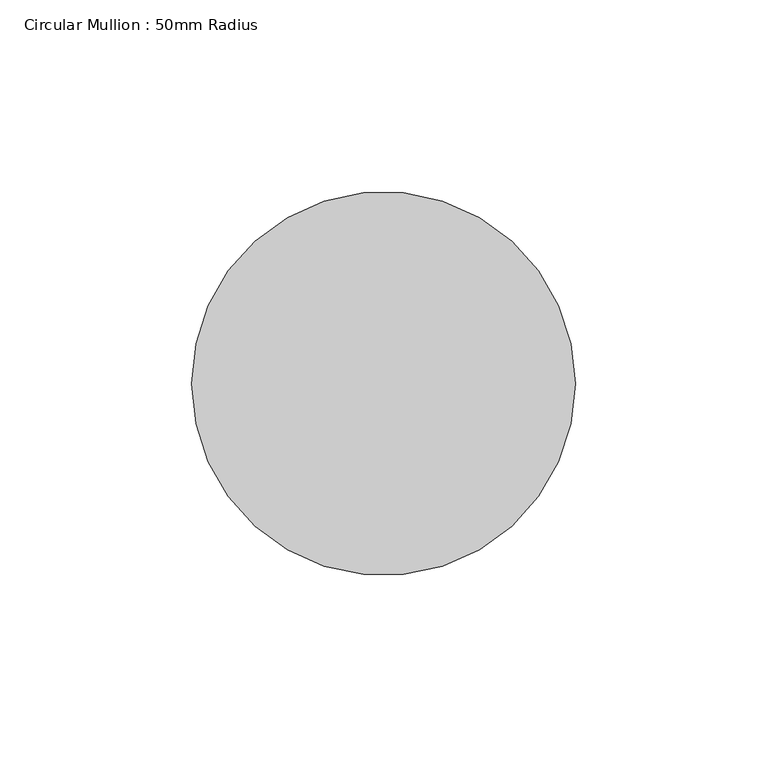
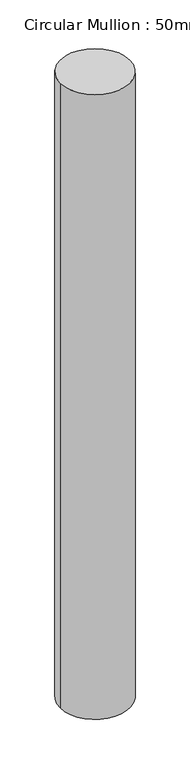
"""IFC4 building model written with IfcOpenShell, lengths in millimetres: member geometry, Circular Mullion : 50mm Radius."""

from ifc_helpers import new_model, si_unit, point, frame, origin, origin_2d, place, context, project, spatial, circle_curve, trimmed, segment, composite_curve, outline, extrude, source, transform, mapped, element, save


def circular_mullion_50mm_radius_479e7c5f(model_context):
    return source(origin(), model_context, "Body", "SweptSolid", [
        extrude(outline(composite_curve([segment(trimmed(circle_curve(origin_2d(), 50.0), [point((50.0, 0.0))], [point((-50.0, 0.0))], False, "CARTESIAN"), True, "CONTINUOUS"), segment(trimmed(circle_curve(origin_2d(), 50.0), [point((-50.0, 0.0))], [point((50.0, 0.0))], False, "CARTESIAN"), True, "CONTINUOUS")], self_intersect=False)), frame((0.0, 0.0, -950.2444532), z_axis=(0.0, 0.0, 1.0), x_axis=(1.0, 0.0, 0.0)), (0.0, 0.0, 1.0), 950.2444532),
    ])


if __name__ == "__main__":
    model = new_model("IFC4")
    model_context = context("Model", 3, world=origin())
    ifc_project = project(units=[si_unit("LENGTHUNIT", "METRE", prefix="MILLI")], contexts=[model_context])
    site = spatial("IfcSite", under=ifc_project)
    building = spatial("IfcBuilding", under=site)
    placement = place(None, origin())
    circular_mullion_50mm_radius_shape = circular_mullion_50mm_radius_479e7c5f(model_context)
    element("IfcMember", 1, ObjectType="Circular Mullion : 50mm Radius", at=placement, inside=building, context=model_context, shape_type="MappedRepresentation", body=[
        mapped(circular_mullion_50mm_radius_shape, transform((0.0, 0.0, 0.0), x_axis=(1.0, 0.0, 0.0), y_axis=(0.0, 1.0, 0.0), z_axis=(0.0, 0.0, 1.0))),
    ])
    save(model, "model.ifc")

# Revit data of these elements
# Type "Circular Mullion : 50mm Radius"
#   built-in parameter 1007350 = 0.164042 (stored number, unit not read)
# Element 1 (IfcMember, "Circular Mullion : 50mm Radius")
#   Materials on its faces: "Aluminium"
# Materials
#   "Aluminium": class "Metal", colour RGB 247 247 247, transparency 0, Description = "Aluminium 6061", Cost = 0
